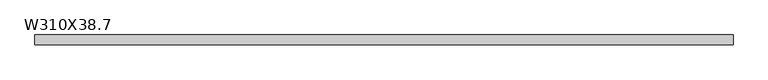
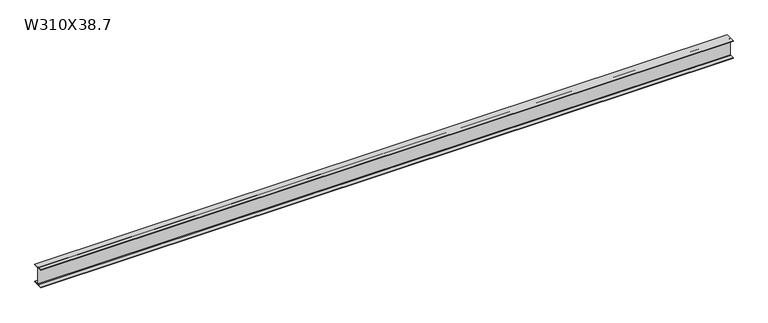
"""IFC4 building model written with IfcOpenShell, lengths in millimetres: beam geometry, M_W Shapes : W310X38.7."""

from ifc_helpers import new_model, si_unit, point, frame, frame_2d, origin, place, context, project, spatial, polyline, circle_curve, trimmed, segment, composite_curve, outline, extrude, source, transform, mapped, element, save


def w310x38_7_02174843(model_context):
    return source(origin(), model_context, "Body", "SweptSolid", [
        extrude(outline(composite_curve([segment(polyline([(82.5, -145.35), (82.5, -155.0), (-82.5, -155.0), (-82.5, -145.35), (-10.57, -145.35)]), True, "CONTINUOUS"), segment(trimmed(circle_curve(frame_2d((-10.57, -137.7)), 7.65), [point((-10.57, -145.35))], [point((-2.92, -137.7))], True, "CARTESIAN"), True, "CONTINUOUS"), segment(polyline([(-2.92, -137.7), (-2.92, 137.7)]), True, "CONTINUOUS"), segment(trimmed(circle_curve(frame_2d((-10.57, 137.7)), 7.65), [point((-2.92, 137.7))], [point((-10.57, 145.35))], True, "CARTESIAN"), True, "CONTINUOUS"), segment(polyline([(-10.57, 145.35), (-82.5, 145.35), (-82.5, 155.0), (82.5, 155.0), (82.5, 145.35), (10.57, 145.35)]), True, "CONTINUOUS"), segment(trimmed(circle_curve(frame_2d((10.57, 137.7)), 7.65), [point((10.57, 145.35))], [point((2.92, 137.7))], True, "CARTESIAN"), True, "CONTINUOUS"), segment(polyline([(2.92, 137.7), (2.92, -137.7)]), True, "CONTINUOUS"), segment(trimmed(circle_curve(frame_2d((10.57, -137.7)), 7.65), [point((2.92, -137.7))], [point((10.57, -145.35))], True, "CARTESIAN"), True, "CONTINUOUS"), segment(polyline([(10.57, -145.35), (82.5, -145.35)]), True, "CONTINUOUS")], self_intersect=False)), frame((-5640.4, 0.0, 0.0), z_axis=(1.0, 0.0, 0.0), x_axis=(0.0, 1.0, 0.0)), (0.0, 0.0, 1.0), 11425.2),
    ])


if __name__ == "__main__":
    model = new_model("IFC4")
    model_context = context("Model", 3, world=origin())
    ifc_project = project(units=[si_unit("LENGTHUNIT", "METRE", prefix="MILLI")], contexts=[model_context])
    site = spatial("IfcSite", under=ifc_project)
    building = spatial("IfcBuilding", under=site)
    placement = place(None, origin())
    w310x38_7_shape = w310x38_7_02174843(model_context)
    element("IfcBeam", 1, ObjectType="M_W Shapes : W310X38.7", at=placement, inside=building, context=model_context, shape_type="MappedRepresentation", body=[
        mapped(w310x38_7_shape, transform((0.0, 0.0, 0.0), x_axis=(1.0, 0.0, 0.0), y_axis=(0.0, 1.0, 0.0), z_axis=(0.0, 0.0, 1.0))),
    ])
    save(model, "model.ifc")

# Revit data of these elements
# Type "M_W Shapes : W310X38.7"
#   Section Name Key = "W12x26"
#   Width = 165 mm
#   Web Thickness = 5.84 mm
#   Web Fillet = 7.65 mm
#   Warping Constant = 163000 cm⁶
#   Torsional Moment of Inertia = 12.5 cm⁴
#   Section Area = 49.4 cm²
#   Plastic Modulus weak axis = 0.00473217 (stored number, unit not read)
#   Plastic Modulus strong axis = 0.0215419 (stored number, unit not read)
#   Perimeter = 1.25 m²/m
#   Nominal Weight = 379.516 N/m
#   Moment of Inertia weak axis = 720 cm⁴
#   Moment of Inertia strong axis = 8490 cm⁴
#   Height = 310 mm
#   Flange Thickness = 9.65 mm
#   Elastic Modulus weak axis = 0.00309003 (stored number, unit not read)
#   Elastic Modulus strong axis = 0.0193171 (stored number, unit not read)
#   Centroid Vertical = 155 mm
#   Centroid Horizontal = 82.5 mm
#   Length [instance default] = 1.5 m
#   Structural Material [instance default] = Steel, 45-345
#   Assembly Code = ""
# Element 1 (IfcBeam, "M_W Shapes : W310X38.7")
#   Materials on its faces: "Steel, 45-345"
# Materials
#   "Steel, 45-345": class "Metal", colour RGB 189 187 185, transparency 0, Description = "Steel 345 MPa", Cost = 0
